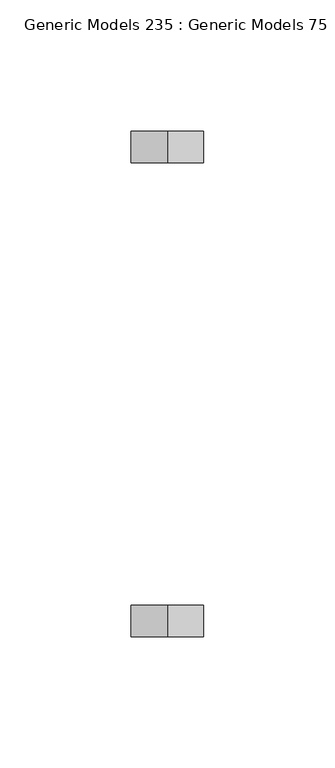
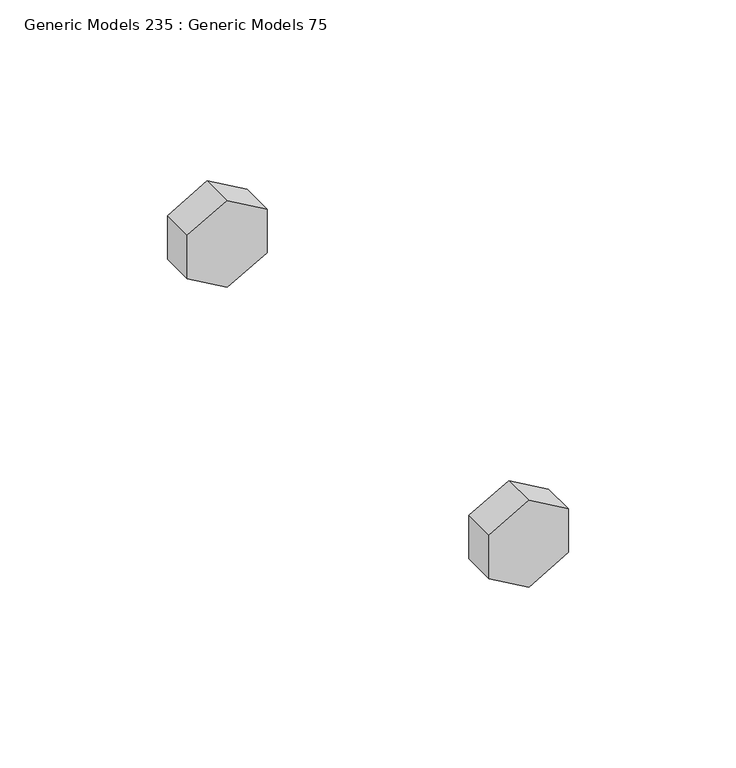
"""IFC4 building model written with IfcOpenShell, lengths in millimetres: proxy geometry, Generic Models 235 : Generic Models 75."""

from ifc_helpers import new_model, si_unit, frame, origin, place, context, project, spatial, polyline, outline, extrude, source, transform, mapped, element, save


def generic_models_235_generic_models_75_2b3cabf5(model_context):
    return source(origin(), model_context, "Body", "SweptSolid", [
        extrude(outline(polyline([(269298.5462802, 31975.9942029), (269282.7097067, 31975.9942029), (269274.79142, 31989.7090778), (269282.7097067, 32003.4239528), (269298.5462802, 32003.4239528), (269306.464567, 31989.7090778), (269298.5462802, 31975.9942029)])), frame((0.0, 35373.9582942, 0.0), z_axis=(0.0, 1.0, 0.0), x_axis=(0.0, 0.0, 1.0)), (0.0, 0.0, 1.0), 11.90625),
        extrude(outline(polyline([(269298.5462802, 31975.9942029), (269282.7097067, 31975.9942029), (269274.79142, 31989.7090778), (269282.7097067, 32003.4239528), (269298.5462802, 32003.4239528), (269306.464567, 31989.7090778), (269298.5462802, 31975.9942029)])), frame((0.0, 35193.7770442, 0.0), z_axis=(0.0, 1.0, 0.0), x_axis=(0.0, 0.0, 1.0)), (0.0, 0.0, 1.0), 11.90625),
    ])


if __name__ == "__main__":
    model = new_model("IFC4")
    model_context = context("Model", 3, world=origin())
    ifc_project = project(units=[si_unit("LENGTHUNIT", "METRE", prefix="MILLI")], contexts=[model_context])
    site = spatial("IfcSite", under=ifc_project)
    building = spatial("IfcBuilding", under=site)
    placement = place(None, origin())
    generic_models_235_generic_models_75_shape = generic_models_235_generic_models_75_2b3cabf5(model_context)
    element("IfcBuildingElementProxy", 1, Name="Generic Models 235 : Generic Models 75", ObjectType="Generic Models 235 : Generic Models 75", at=placement, inside=building, context=model_context, shape_type="MappedRepresentation", body=[
        mapped(generic_models_235_generic_models_75_shape, transform((0.0, 0.0, 0.0), x_axis=(1.0, 0.0, 0.0), y_axis=(0.0, 1.0, 0.0), z_axis=(0.0, 0.0, 1.0))),
    ])
    save(model, "model.ifc")

# Revit data of these elements
# Element 1 (IfcBuildingElementProxy, "Generic Models 235 : Generic Models 75")
#   Materials on its faces: "3/4\" GALV. THRU BOLTS"
# Materials
#   "3/4\" GALV. THRU BOLTS": class "Generic", colour RGB 105 69 171, transparency 0, Cost = 0
